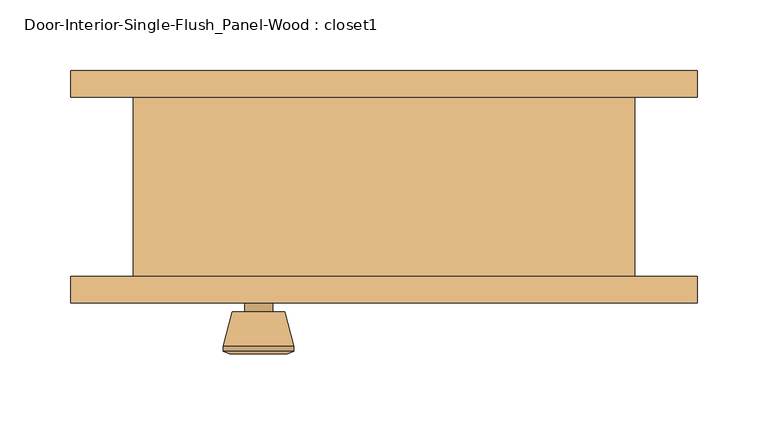
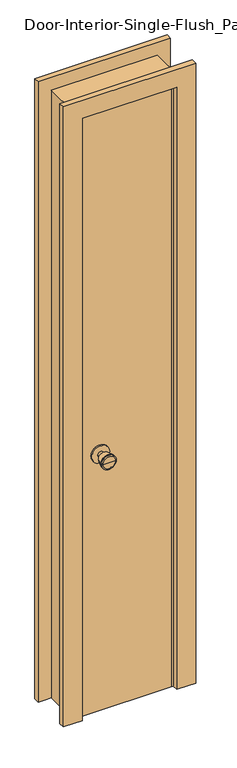
"""IFC4 building model written with IfcOpenShell, lengths in millimetres: door geometry, Door-Interior-Single-Flush_Panel-Wood : closet1."""

from ifc_helpers import new_model, si_unit, point, frame, frame_2d, origin, origin_with_axes, place, context, project, spatial, polyline, circle_curve, trimmed, segment, composite_curve, outline, extrude, faceted_brep, source, transform, mapped, element, save
from ifc_brep_helpers import plane_surface, cylinder_surface, revolved_surface, advanced_brep


def door_interior_single_flush_panel_wood_closet1_fab5e597(model_context):
    return source(origin(), model_context, "Body", "SolidModel", [
        advanced_brep(
        [(-88.9, -19.4, 914.4), (-98.9, -19.4, 914.4), (-78.9, -19.4, 914.4), (-68.4241324, 29.6, 914.4), (-109.3758676, 29.6, 914.4), (-88.9, 29.6, 914.4), (-63.9, 27.7721319, 914.4), (-113.9, 27.7721319, 914.4), (-63.9, 24.3084537, 914.4), (-113.9, 24.3084537, 914.4), (-70.263764, -0.4, 914.4), (-107.536236, -0.4, 914.4), (-78.9, -0.4, 914.4), (-98.9, -0.4, 914.4)],
        [
            (0, 1),
            (1, 2, circle_curve(frame((-88.9, -19.4, 914.4), z_axis=(0.0, -1.0, 0.0), x_axis=(-1.0, 0.0, 0.0)), 10.0)),
            (2, 0),
            (2, 1, circle_curve(frame((-88.9, -19.4, 914.4), z_axis=(0.0, -1.0, 0.0), x_axis=(-1.0, 0.0, 0.0)), 10.0)),
            (3, 4, circle_curve(frame((-88.9, 29.6, 914.4), z_axis=(0.0, 1.0, 0.0), x_axis=(-1.0, 0.0, 0.0)), 20.4758676)),
            (4, 5),
            (5, 3),
            (4, 3, circle_curve(frame((-88.9, 29.6, 914.4), z_axis=(0.0, 1.0, 0.0), x_axis=(-1.0, 0.0, 0.0)), 20.4758676)),
            (6, 7, circle_curve(frame((-88.9, 27.7721319, 914.4), z_axis=(0.0, 1.0, 0.0), x_axis=(-1.0, 0.0, 0.0)), 25.0)),
            (7, 4),
            (3, 6),
            (7, 6, circle_curve(frame((-88.9, 27.7721319, 914.4), z_axis=(0.0, 1.0, 0.0), x_axis=(-1.0, 0.0, 0.0)), 25.0)),
            (8, 9, circle_curve(frame((-88.9, 24.3084537, 914.4), z_axis=(0.0, 1.0, 0.0), x_axis=(-1.0, 0.0, 0.0)), 25.0)),
            (9, 7),
            (6, 8),
            (9, 8, circle_curve(frame((-88.9, 24.3084537, 914.4), z_axis=(0.0, 1.0, 0.0), x_axis=(-1.0, 0.0, 0.0)), 25.0)),
            (10, 11, circle_curve(frame((-88.9, -0.4, 914.4), z_axis=(0.0, 1.0, 0.0), x_axis=(-1.0, 0.0, 0.0)), 18.636236)),
            (11, 9),
            (8, 10),
            (11, 10, circle_curve(frame((-88.9, -0.4, 914.4), z_axis=(0.0, 1.0, 0.0), x_axis=(-1.0, 0.0, 0.0)), 18.636236)),
            (12, 13, circle_curve(frame((-88.9, -0.4, 914.4), z_axis=(0.0, 1.0, 0.0), x_axis=(-1.0, 0.0, 0.0)), 10.0)),
            (13, 11),
            (10, 12),
            (13, 12, circle_curve(frame((-88.9, -0.4, 914.4), z_axis=(0.0, 1.0, 0.0), x_axis=(-1.0, 0.0, 0.0)), 10.0)),
            (1, 13),
            (12, 2),
        ],
        [
            plane_surface(frame((-88.9, -19.4, 914.4), z_axis=(0.0, -1.0, 0.0), x_axis=(-1.0, 0.0, 0.0))),
            plane_surface(frame((-88.9, 29.6, 914.4), z_axis=(0.0, 1.0, 0.0), x_axis=(-1.0, 0.0, 0.0))),
            revolved_surface(polyline([(-109.3758676, 29.6, 914.4), (-113.9, 27.7721319, 914.4)]), (-88.9, -19.4, 914.4), (0.0, -1.0, 0.0)),
            cylinder_surface(frame((-88.9, -19.4, 914.4), z_axis=(0.0, -1.0, 0.0), x_axis=(-1.0, 0.0, 0.0)), 25.0),
            revolved_surface(polyline([(-113.9, 24.3084537, 914.4), (-107.536236, -0.4, 914.4)]), (-88.9, -19.4, 914.4), (0.0, -1.0, 0.0)),
            plane_surface(frame((-88.9, -0.4, 914.4), z_axis=(0.0, -1.0, 0.0), x_axis=(-1.0, 0.0, 0.0))),
            cylinder_surface(frame((-88.9, -19.4, 914.4), z_axis=(0.0, -1.0, 0.0), x_axis=(-1.0, 0.0, 0.0)), 10.0),
        ],
        [
            (0, [[1, 2, 3]]),
            (0, [[-3, 4, -1]]),
            (1, [[5, 6, 7]]),
            (1, [[8, -7, -6]]),
            (2, [[9, 10, -5, 11]]),
            (2, [[12, -11, -8, -10]]),
            (3, [[13, 14, -9, 15]]),
            (3, [[16, -15, -12, -14]]),
            (4, [[17, 18, -13, 19]]),
            (4, [[20, -19, -16, -18]]),
            (5, [[21, 22, -17, 23]]),
            (5, [[24, -23, -20, -22]]),
            (6, [[-2, 25, -21, 26]]),
            (6, [[-4, -26, -24, -25]]),
        ],
    ),
        extrude(outline(composite_curve([segment(trimmed(circle_curve(frame_2d((914.4, -88.9)), 30.0), [point((914.4, -118.9))], [point((914.4, -58.9))], False, "CARTESIAN"), True, "CONTINUOUS"), segment(trimmed(circle_curve(frame_2d((914.4, -88.9)), 30.0), [point((914.4, -58.9))], [point((914.4, -118.9))], False, "CARTESIAN"), True, "CONTINUOUS")], self_intersect=False)), frame((0.0, -25.4, 0.0), z_axis=(0.0, 1.0, 0.0), x_axis=(0.0, 0.0, 1.0)), (0.0, 0.0, 1.0), 6.0),
        advanced_brep(
        [(-88.9, -66.325, 914.4), (-78.9, -66.325, 914.4), (-98.9, -66.325, 914.4), (-68.4241324, -115.325, 914.4), (-88.9, -115.325, 914.4), (-109.3758676, -115.325, 914.4), (-63.9, -113.4971319, 914.4), (-113.9, -113.4971319, 914.4), (-63.9, -110.0334537, 914.4), (-113.9, -110.0334537, 914.4), (-70.263764, -85.325, 914.4), (-107.536236, -85.325, 914.4), (-78.9, -85.325, 914.4), (-98.9, -85.325, 914.4)],
        [
            (0, 1),
            (1, 2, circle_curve(frame((-88.9, -66.325, 914.4), z_axis=(0.0, 1.0, 0.0), x_axis=(-1.0, 0.0, 0.0)), 10.0)),
            (2, 0),
            (2, 1, circle_curve(frame((-88.9, -66.325, 914.4), z_axis=(0.0, 1.0, 0.0), x_axis=(-1.0, 0.0, 0.0)), 10.0)),
            (3, 4),
            (4, 5),
            (5, 3, circle_curve(frame((-88.9, -115.325, 914.4), z_axis=(0.0, -1.0, 0.0), x_axis=(-1.0, 0.0, 0.0)), 20.4758676)),
            (3, 5, circle_curve(frame((-88.9, -115.325, 914.4), z_axis=(0.0, -1.0, 0.0), x_axis=(-1.0, 0.0, 0.0)), 20.4758676)),
            (6, 3),
            (5, 7),
            (7, 6, circle_curve(frame((-88.9, -113.4971319, 914.4), z_axis=(0.0, -1.0, 0.0), x_axis=(-1.0, 0.0, 0.0)), 25.0)),
            (6, 7, circle_curve(frame((-88.9, -113.4971319, 914.4), z_axis=(0.0, -1.0, 0.0), x_axis=(-1.0, 0.0, 0.0)), 25.0)),
            (8, 6),
            (7, 9),
            (9, 8, circle_curve(frame((-88.9, -110.0334537, 914.4), z_axis=(0.0, -1.0, 0.0), x_axis=(-1.0, 0.0, 0.0)), 25.0)),
            (8, 9, circle_curve(frame((-88.9, -110.0334537, 914.4), z_axis=(0.0, -1.0, 0.0), x_axis=(-1.0, 0.0, 0.0)), 25.0)),
            (10, 8),
            (9, 11),
            (11, 10, circle_curve(frame((-88.9, -85.325, 914.4), z_axis=(0.0, -1.0, 0.0), x_axis=(-1.0, 0.0, 0.0)), 18.636236)),
            (10, 11, circle_curve(frame((-88.9, -85.325, 914.4), z_axis=(0.0, -1.0, 0.0), x_axis=(-1.0, 0.0, 0.0)), 18.636236)),
            (12, 10),
            (11, 13),
            (13, 12, circle_curve(frame((-88.9, -85.325, 914.4), z_axis=(0.0, -1.0, 0.0), x_axis=(-1.0, 0.0, 0.0)), 10.0)),
            (12, 13, circle_curve(frame((-88.9, -85.325, 914.4), z_axis=(0.0, -1.0, 0.0), x_axis=(-1.0, 0.0, 0.0)), 10.0)),
            (1, 12),
            (13, 2),
        ],
        [
            plane_surface(frame((-88.9, -66.325, 914.4), z_axis=(0.0, 1.0, 0.0), x_axis=(-1.0, 0.0, 0.0))),
            plane_surface(frame((-88.9, -115.325, 914.4), z_axis=(0.0, -1.0, 0.0), x_axis=(-1.0, 0.0, 0.0))),
            revolved_surface(polyline([(-109.3758676, -115.325, 914.4), (-113.9, -113.4971319, 914.4)]), (-88.9, -66.325, 914.4), (0.0, 1.0, 0.0)),
            cylinder_surface(frame((-88.9, -66.325, 914.4), z_axis=(0.0, 1.0, 0.0), x_axis=(-1.0, 0.0, 0.0)), 25.0),
            revolved_surface(polyline([(-113.9, -110.0334537, 914.4), (-107.536236, -85.325, 914.4)]), (-88.9, -66.325, 914.4), (0.0, 1.0, 0.0)),
            plane_surface(frame((-88.9, -85.325, 914.4), z_axis=(0.0, 1.0, 0.0), x_axis=(-1.0, 0.0, 0.0))),
            cylinder_surface(frame((-88.9, -66.325, 914.4), z_axis=(0.0, 1.0, 0.0), x_axis=(-1.0, 0.0, 0.0)), 10.0),
        ],
        [
            (0, [[1, 2, 3]]),
            (0, [[-3, 4, -1]]),
            (1, [[5, 6, 7]]),
            (1, [[-6, -5, 8]]),
            (2, [[9, -7, 10, 11]]),
            (2, [[-10, -8, -9, 12]]),
            (3, [[13, -11, 14, 15]]),
            (3, [[-14, -12, -13, 16]]),
            (4, [[17, -15, 18, 19]]),
            (4, [[-18, -16, -17, 20]]),
            (5, [[21, -19, 22, 23]]),
            (5, [[-22, -20, -21, 24]]),
            (6, [[25, -23, 26, -2]]),
            (6, [[-26, -24, -25, -4]]),
        ],
    ),
        extrude(outline(composite_curve([segment(trimmed(circle_curve(frame_2d((914.4, -88.9)), 30.0), [point((914.4, -118.9))], [point((914.4, -58.9))], False, "CARTESIAN"), True, "CONTINUOUS"), segment(trimmed(circle_curve(frame_2d((914.4, -88.9)), 30.0), [point((914.4, -58.9))], [point((914.4, -118.9))], False, "CARTESIAN"), True, "CONTINUOUS")], self_intersect=False)), frame((0.0, -66.325, 0.0), z_axis=(0.0, 1.0, 0.0), x_axis=(0.0, 0.0, 1.0)), (0.0, 0.0, 1.0), 6.0),
        extrude(outline(polyline([(152.4, -25.4), (152.4, -60.325), (-152.4, -60.325), (-152.4, -25.4), (152.4, -25.4)])), origin_with_axes(), (0.0, 0.0, 1.0), 2133.6),
        faceted_brep([(177.8, -60.325, 0.0), (152.4, -60.325, 0.0), (152.4, -25.4, 0.0), (139.7, -25.4, 0.0), (139.7, 9.525, 0.0), (152.4, 9.525, 0.0), (152.4, 66.675, 0.0), (177.8, 66.675, 0.0), (177.8, 66.675, 2159.0), (177.8, -60.325, 2159.0), (152.4, 66.675, 2133.6), (-152.4, 66.675, 2133.6), (-152.4, 66.675, 0.0), (-177.8, 66.675, 0.0), (-177.8, 66.675, 2159.0), (152.4, 9.525, 2133.6), (139.7, 9.525, 2120.9), (-139.7, 9.525, 2120.9), (-139.7, 9.525, 0.0), (-152.4, 9.525, 0.0), (-152.4, 9.525, 2133.6), (139.7, -25.4, 2120.9), (152.4, -25.4, 2133.6), (-152.4, -25.4, 2133.6), (-152.4, -25.4, 0.0), (-139.7, -25.4, 0.0), (-139.7, -25.4, 2120.9), (152.4, -60.325, 2133.6), (-177.8, -60.325, 2159.0), (-177.8, -60.325, 0.0), (-152.4, -60.325, 0.0), (-152.4, -60.325, 2133.6)], [[[0, 1, 2, 3, 4, 5, 6, 7]], [[7, 8, 9, 0]], [[6, 10, 11, 12, 13, 14, 8, 7]], [[5, 15, 10, 6]], [[4, 16, 17, 18, 19, 20, 15, 5]], [[3, 21, 16, 4]], [[2, 22, 23, 24, 25, 26, 21, 3]], [[1, 27, 22, 2]], [[0, 9, 28, 29, 30, 31, 27, 1]], [[8, 14, 28, 9]], [[15, 20, 11, 10]], [[21, 26, 17, 16]], [[27, 31, 23, 22]], [[29, 13, 12, 19, 18, 25, 24, 30]], [[14, 13, 29, 28]], [[20, 19, 12, 11]], [[26, 25, 18, 17]], [[31, 30, 24, 23]]]),
        extrude(outline(polyline([(0.0, 222.25), (2203.45, 222.25), (2203.45, -222.25), (0.0, -222.25), (0.0, -158.75), (2139.95, -158.75), (2139.95, 158.75), (0.0, 158.75), (0.0, 222.25)])), frame((0.0, 66.675, 0.0), z_axis=(0.0, 1.0, 0.0), x_axis=(0.0, 0.0, 1.0)), (0.0, 0.0, 1.0), 19.05),
        extrude(outline(polyline([(0.0, 222.25), (2203.45, 222.25), (2203.45, -222.25), (0.0, -222.25), (0.0, -158.75), (2139.95, -158.75), (2139.95, 158.75), (0.0, 158.75), (0.0, 222.25)])), frame((0.0, -79.375, 0.0), z_axis=(0.0, 1.0, 0.0), x_axis=(0.0, 0.0, 1.0)), (0.0, 0.0, 1.0), 19.05),
    ])


if __name__ == "__main__":
    model = new_model("IFC4")
    model_context = context("Model", 3, world=origin())
    ifc_project = project(units=[si_unit("LENGTHUNIT", "METRE", prefix="MILLI")], contexts=[model_context])
    site = spatial("IfcSite", under=ifc_project)
    building = spatial("IfcBuilding", under=site)
    placement = place(None, origin())
    door_interior_single_flush_panel_wood_closet1_shape = door_interior_single_flush_panel_wood_closet1_fab5e597(model_context)
    element("IfcDoor", 1, ObjectType="Door-Interior-Single-Flush_Panel-Wood : closet1", at=placement, inside=building, context=model_context, shape_type="MappedRepresentation", body=[
        mapped(door_interior_single_flush_panel_wood_closet1_shape, transform((0.0, 0.0, 0.0), x_axis=(1.0, 0.0, 0.0), y_axis=(0.0, 1.0, 0.0), z_axis=(0.0, 0.0, 1.0))),
    ])
    save(model, "model.ifc")

# Revit data of these elements
# Type "Door-Interior-Single-Flush_Panel-Wood : closet1"
#   Type Mark = "w"
#   Assembly Code = "C1020300"
#   Analytic Construction = "Wooden"
#   Thickness = 0' - 1 3/8"
#   Thermal Resistance (R) = 0.455703 (m²·K)/W
#   Swing Angle [instance default] = 90.00°
#   Rough Width = 1' - 2"
#   Rough Height = 7' - 1"
#   Height = 7' - 0"
#   Width = 1' - 0"
#   Heat Transfer Coefficient (U) = 2.19465 W/(m²·K)
#   Trim Material = Cherry
#   Panel Material = Cherry
#   Frame Material = Cherry
#   Door Handle Material = Aluminum
#   Visual Light Transmittance = 0
#   Solar Heat Gain Coefficient = 0
#   Wall Closure = (empty or 0)
#   Function = (empty or 0)
# Element 1 (IfcDoor, "Door-Interior-Single-Flush_Panel-Wood : closet1")
#   Materials on its faces: "Cherry", "Aluminum"
# Materials
#   "Cherry": class "Wood", colour RGB 154 107 61, transparency 0, Description = "Prunus Serotina", Cost = 0
#   "Aluminum": class "Metal", colour RGB 244 244 244, transparency 0, Description = "Aluminum 6061", Cost = 0
